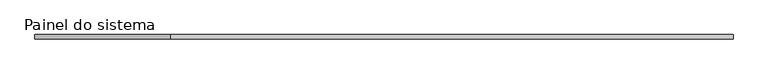
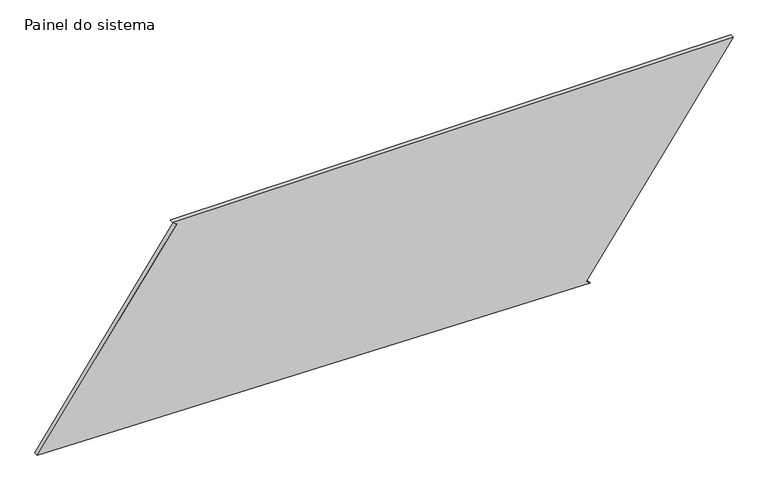
"""IFC4 building model written with IfcOpenShell, lengths in millimetres: plate geometry, Painel do sistema : Envidraçado."""

from ifc_helpers import new_model, si_unit, frame, origin, place, context, project, spatial, polyline, outline, extrude, source, transform, mapped, element, save


def painel_do_sistema_cb45a691(model_context):
    return source(origin(), model_context, "Body", "SweptSolid", [
        extrude(outline(polyline([(0.0, 1141.2572669), (14.4529738, 1120.8584544), (1168.4111121, 1938.4612838), (1168.4111121, -1183.8147657), (1153.9581383, -1163.4159533), (60.0653158, -1938.4612838), (0.0, 1141.2572669)])), frame((0.0, 24.5, 0.0), z_axis=(0.0, 1.0, 0.0), x_axis=(0.0, 0.0, 1.0)), (0.0, 0.0, 1.0), 25.0),
    ])


if __name__ == "__main__":
    model = new_model("IFC4")
    model_context = context("Model", 3, world=origin())
    ifc_project = project(units=[si_unit("LENGTHUNIT", "METRE", prefix="MILLI")], contexts=[model_context])
    site = spatial("IfcSite", under=ifc_project)
    building = spatial("IfcBuilding", under=site)
    placement = place(None, origin())
    painel_do_sistema_shape = painel_do_sistema_cb45a691(model_context)
    element("IfcPlate", 1, ObjectType="Painel do sistema : Envidraçado", at=placement, inside=building, context=model_context, shape_type="MappedRepresentation", body=[
        mapped(painel_do_sistema_shape, transform((0.0, 0.0, 0.0), x_axis=(1.0, 0.0, 0.0), y_axis=(0.0, 1.0, 0.0), z_axis=(0.0, 0.0, 1.0))),
    ])
    save(model, "model.ifc")

# Revit data of these elements
# Type "Painel do sistema : Envidraçado"
#   Construction Type Id = "GSP4R"
#   Analytic Construction = "Vidraça única Pilkington 1/8 pol"
#   Visual Light Transmittance = 0.9
#   Solar Heat Gain Coefficient = 0.86
#   Heat Transfer Coefficient (U) = 6.7069 W/(m²·K)
# Element 1 (IfcPlate, "Painel do sistema : Envidraçado")
#   Materials on its faces: "Vidro"
# Materials
#   "Vidro": class "Vidro", colour RGB 0 128 192, transparency 0.9, Description = "Vidro de sílica", Cost = 0
